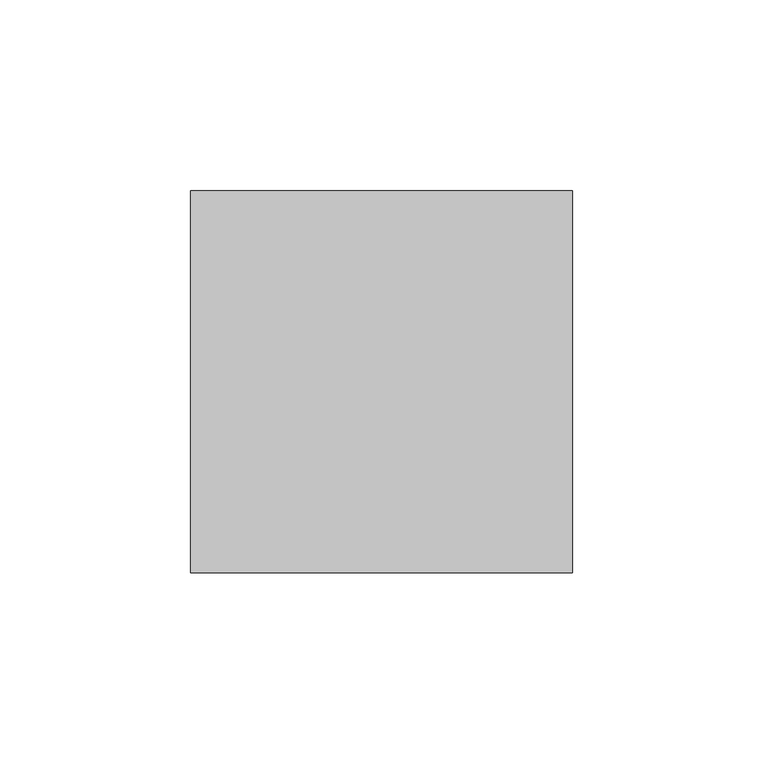
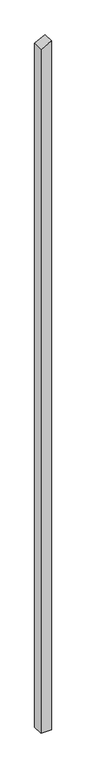
"""IFC4 building model written with IfcOpenShell, lengths in millimetres: column geometry, Holzstütze 160106 : Holzstütze 160106."""

from ifc_helpers import new_model, si_unit, frame, origin, place, context, project, spatial, polyline, outline, extrude, source, transform, mapped, element, save


def column_380c84c3(model_context):
    return source(origin(), model_context, "Body", "SweptSolid", [
        extrude(outline(polyline([(-500.0, 157297.7593015), (-500.0, 157397.7593015), (6396.6643707, 157397.7593015), (6345.7118258, 157297.7593015), (-500.0, 157297.7593015)])), frame((0.0, 33138.3551606, 0.0), z_axis=(0.0, 1.0, 0.0), x_axis=(0.0, 0.0, 1.0)), (0.0, 0.0, 1.0), 100.0),
    ])


if __name__ == "__main__":
    model = new_model("IFC4")
    model_context = context("Model", 3, world=origin())
    ifc_project = project(units=[si_unit("LENGTHUNIT", "METRE", prefix="MILLI")], contexts=[model_context])
    site = spatial("IfcSite", under=ifc_project)
    building = spatial("IfcBuilding", under=site)
    placement = place(None, origin())
    column_shape = column_380c84c3(model_context)
    element("IfcColumn", 1, ObjectType="Holzstütze 160106 : Holzstütze 160106", at=placement, inside=building, context=model_context, shape_type="MappedRepresentation", body=[
        mapped(column_shape, transform((0.0, 0.0, 0.0), x_axis=(1.0, 0.0, 0.0), y_axis=(0.0, 1.0, 0.0), z_axis=(0.0, 0.0, 1.0))),
    ])
    save(model, "model.ifc")

# Revit data of these elements
# Type "Holzstütze 160106 : Holzstütze 160106"
#   Abrechnungsart = "m"
#   Allright_Bauteil_ID = "0152St 0000143342"
#   Bezeichnung = "Holzstütze"
#   Codetext = "ST-HOLZ\\"
#   Gewerk = "Zimmer- und Holzbauarbeiten"
#   Material = "Holz"
#   Objektname = "Stütze"
#   NameOverride = "Holzstütze"
#   Reference = "Holzstütze"
#   Status = "NEW"
#   ThermalTransmittance = 0.0000 BTU/(h·ft²·°F)
#   Roll = 0.00°
#   Slope = 0.00°
#   2D Interaktion = yes
#   IsExternal = yes
#   LoadBearing = yes
# Element 1 (IfcColumn, "Holzstütze 160106 : Holzstütze 160106")
#   Materials on its faces: "holzschalung"
# Materials
#   "holzschalung": class "Unassigned", colour RGB 128 128 128, transparency 0
